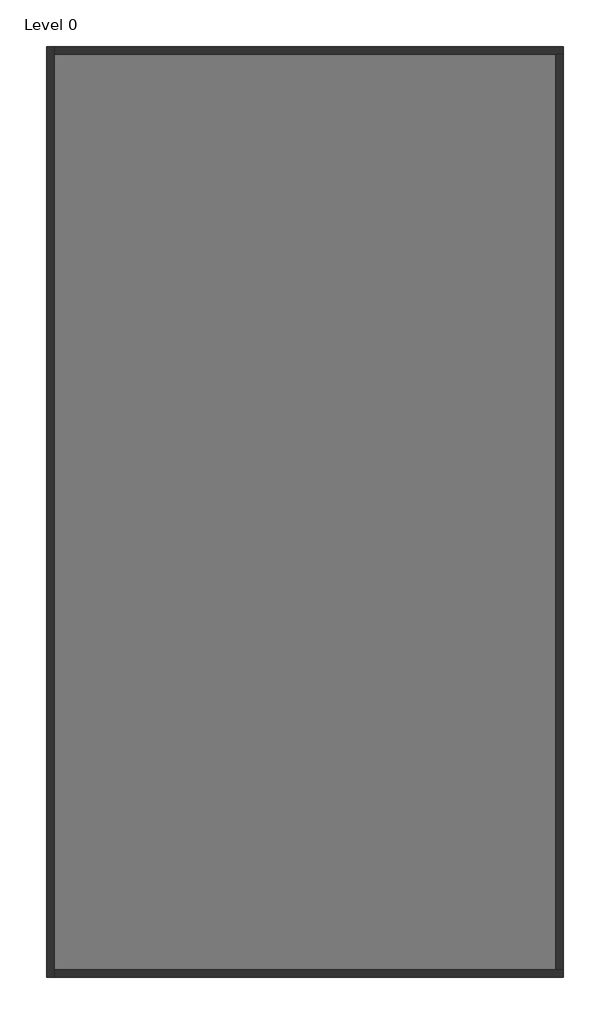
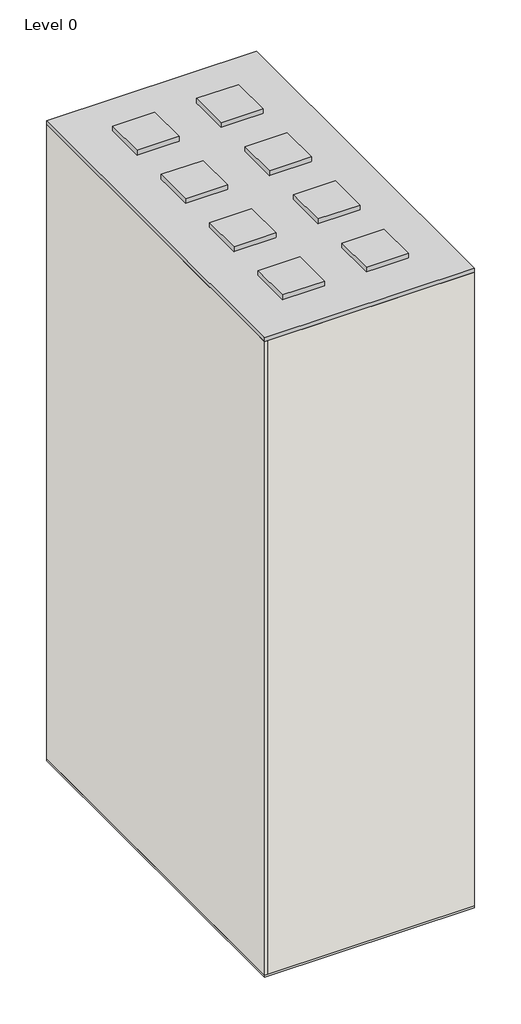
# One storey: 4 walls, 1 proxy, 1 slab.
"""IFC4 building model written with IfcOpenShell, lengths in millimetres."""

from ifc_helpers import new_model, si_unit, frame, origin, origin_with_axes, place, context, project, spatial, polyline, outline, extrude, faceted_brep, element, save

model = new_model("IFC4")

# Units and contexts
model_context = context("Model", 3, world=origin())
ifc_project = project(units=[si_unit("LENGTHUNIT", "METRE", prefix="MILLI")], contexts=[model_context])

# Site, building, storey
site = spatial("IfcSite", under=ifc_project)
building = spatial("IfcBuilding", under=site)
storey = spatial("IfcBuildingStorey", under=building, Name="Level 0", Elevation=100.0)

# Proxy
placement = place(None, origin())
element("IfcBuildingElementProxy", 1, Name="LowUrbanDensityBuilding : LowUrbanDensityBuilding", ObjectType="LowUrbanDensityBuilding : LowUrbanDensityBuilding", at=placement, inside=storey, context=model_context, shape_type="SweptSolid", body=[
    extrude(outline(polyline([(7325.2659446, 3676.2074539), (7325.2659446, -14323.7925461), (-2674.7340554, -14323.7925461), (-2674.7340554, 3676.2074539), (7325.2659446, 3676.2074539)])), origin_with_axes(), (0.0, 0.0, 1.0), 32200.0),
    extrude(outline(polyline([(1325.2659446, 1676.2074539), (1325.2659446, -323.7925461), (-674.7340554, -323.7925461), (-674.7340554, 1676.2074539), (1325.2659446, 1676.2074539)])), frame((0.0, 0.0, 32000.0), z_axis=(0.0, 0.0, 1.0), x_axis=(1.0, 0.0, 0.0)), (0.0, 0.0, 1.0), 445.0),
    extrude(outline(polyline([(3325.2659446, -323.7925461), (3325.2659446, 1676.2074539), (5325.2659446, 1676.2074539), (5325.2659446, -323.7925461), (3325.2659446, -323.7925461)])), frame((0.0, 0.0, 32000.0), z_axis=(0.0, 0.0, 1.0), x_axis=(1.0, 0.0, 0.0)), (0.0, 0.0, 1.0), 445.0),
    extrude(outline(polyline([(1325.2659446, -2323.7925461), (1325.2659446, -4323.7925461), (-674.7340554, -4323.7925461), (-674.7340554, -2323.7925461), (1325.2659446, -2323.7925461)])), frame((0.0, 0.0, 32000.0), z_axis=(0.0, 0.0, 1.0), x_axis=(1.0, 0.0, 0.0)), (0.0, 0.0, 1.0), 445.0),
    extrude(outline(polyline([(3325.2659446, -4323.7925461), (3325.2659446, -2323.7925461), (5325.2659446, -2323.7925461), (5325.2659446, -4323.7925461), (3325.2659446, -4323.7925461)])), frame((0.0, 0.0, 32000.0), z_axis=(0.0, 0.0, 1.0), x_axis=(1.0, 0.0, 0.0)), (0.0, 0.0, 1.0), 445.0),
    extrude(outline(polyline([(-674.7340554, -8323.7925461), (-674.7340554, -6323.7925461), (1325.2659446, -6323.7925461), (1325.2659446, -8323.7925461), (-674.7340554, -8323.7925461)])), frame((0.0, 0.0, 32000.0), z_axis=(0.0, 0.0, 1.0), x_axis=(1.0, 0.0, 0.0)), (0.0, 0.0, 1.0), 445.0),
    extrude(outline(polyline([(3325.2659446, -8323.7925461), (3325.2659446, -6323.7925461), (5325.2659446, -6323.7925461), (5325.2659446, -8323.7925461), (3325.2659446, -8323.7925461)])), frame((0.0, 0.0, 32000.0), z_axis=(0.0, 0.0, 1.0), x_axis=(1.0, 0.0, 0.0)), (0.0, 0.0, 1.0), 445.0),
    extrude(outline(polyline([(-674.7340554, -12323.7925461), (-674.7340554, -10323.7925461), (1325.2659446, -10323.7925461), (1325.2659446, -12323.7925461), (-674.7340554, -12323.7925461)])), frame((0.0, 0.0, 32000.0), z_axis=(0.0, 0.0, 1.0), x_axis=(1.0, 0.0, 0.0)), (0.0, 0.0, 1.0), 445.0),
    extrude(outline(polyline([(5325.2659446, -10323.7925461), (5325.2659446, -12323.7925461), (3325.2659446, -12323.7925461), (3325.2659446, -10323.7925461), (5325.2659446, -10323.7925461)])), frame((0.0, 0.0, 32000.0), z_axis=(0.0, 0.0, 1.0), x_axis=(1.0, 0.0, 0.0)), (0.0, 0.0, 1.0), 445.0),
])

# Slab
element("IfcSlab", 2, ObjectType="Floor-Concrete_100Con", at=placement, inside=storey, context=model_context, shape_type="SweptSolid", body=[
    extrude(outline(polyline([(7325.2659446, 3676.2074539), (7325.2659446, -14323.7925461), (-2674.7340554, -14323.7925461), (-2674.7340554, 3676.2074539), (7325.2659446, 3676.2074539)])), origin_with_axes(), (0.0, 0.0, 1.0), 100.0),
])

# Walls
element("IfcWall", 3, ObjectType="Wall-Ext_25Rdr-100Blk-19P", at=placement, inside=storey, context=model_context, shape_type="Brep", body=[
    faceted_brep([(-2674.7340554, 3676.2074539, 100.0), (-2674.7340554, -14323.7925461, 100.0), (-2674.7340554, -14323.7925461, 32000.0), (-2674.7340554, 3676.2074539, 32000.0), (-2530.4340554, 3676.2074539, 100.0), (-2530.4340554, 3676.2074539, 32000.0), (-2530.4340554, 3531.9074539, 32000.0), (-2530.4340554, -14179.4925461, 32000.0), (-2530.4340554, -14323.7925461, 32000.0), (-2530.4340554, -14323.7925461, 100.0), (-2530.4340554, -14179.4925461, 100.0), (-2530.4340554, 3531.9074539, 100.0)], [[[0, 1, 2, 3]], [[4, 5, 6, 7, 8, 9, 10, 11]], [[1, 0, 4, 11, 10, 9]], [[3, 2, 8, 7, 6, 5]], [[2, 1, 9, 8]], [[0, 3, 5, 4]]]),
])
element("IfcWall", 4, ObjectType="Wall-Ext_25Rdr-100Blk-19P", at=placement, inside=storey, context=model_context, shape_type="Brep", body=[
    faceted_brep([(-2530.4340554, -14323.7925461, 100.0), (7325.2659446, -14323.7925461, 100.0), (7325.2659446, -14323.7925461, 32000.0), (-2530.4340554, -14323.7925461, 32000.0), (-2530.4340554, -14179.4925461, 100.0), (-2530.4340554, -14179.4925461, 32000.0), (7180.9659446, -14179.4925461, 32000.0), (7325.2659446, -14179.4925461, 32000.0), (7325.2659446, -14179.4925461, 100.0), (7180.9659446, -14179.4925461, 100.0)], [[[0, 1, 2, 3]], [[4, 5, 6, 7, 8, 9]], [[1, 0, 4, 9, 8]], [[3, 2, 7, 6, 5]], [[0, 3, 5, 4]], [[2, 1, 8, 7]]]),
])
element("IfcWall", 5, ObjectType="Wall-Ext_25Rdr-100Blk-19P", at=placement, inside=storey, context=model_context, shape_type="Brep", body=[
    faceted_brep([(7325.2659446, 3676.2074539, 100.0), (-2530.4340554, 3676.2074539, 100.0), (-2530.4340554, 3676.2074539, 32000.0), (7325.2659446, 3676.2074539, 32000.0), (7325.2659446, 3531.9074539, 100.0), (7325.2659446, 3531.9074539, 32000.0), (7180.9659446, 3531.9074539, 32000.0), (-2530.4340554, 3531.9074539, 32000.0), (-2530.4340554, 3531.9074539, 100.0), (7180.9659446, 3531.9074539, 100.0)], [[[0, 1, 2, 3]], [[4, 5, 6, 7, 8, 9]], [[1, 0, 4, 9, 8]], [[3, 2, 7, 6, 5]], [[2, 1, 8, 7]], [[0, 3, 5, 4]]]),
])
element("IfcWall", 6, ObjectType="Wall-Ext_25Rdr-100Blk-19P", at=placement, inside=storey, context=model_context, shape_type="SweptSolid", body=[
    extrude(outline(polyline([(7325.2659446, 3531.9074539), (7325.2659446, -14179.4925461), (7180.9659446, -14179.4925461), (7180.9659446, 3531.9074539), (7325.2659446, 3531.9074539)])), frame((0.0, 0.0, 100.0), z_axis=(0.0, 0.0, 1.0), x_axis=(1.0, 0.0, 0.0)), (0.0, 0.0, 1.0), 31900.0),
])

save(model, "model.ifc")

# Revit data of these elements
# Project information
#   Project Issue Date = "Issue Date"
#   Project Status = "Project Status"
#   Client Name = "Owner"
#   Project Address = "Enter address here"
#   Project Name = "Project Name"
#   Project Number = "Project Number"
# Type "Floor-Concrete_100Con"
#   Keynote = "E60/130"
#   Function = 0
#   Layers, outside or top first: 100 mm "Concrete" (function 1)
# Type "Wall-Ext_25Rdr-100Blk-19P"
#   Keynote = "F10"
#   Layers, outside or top first: 25.3 mm "Render, Beige, Smooth" (function 5); 100 mm "Concrete Masonry Units _Low Density" (function 1); 19 mm "Plaster" (function 5)
# Element 1 (IfcBuildingElementProxy, "LowUrbanDensityBuilding : LowUrbanDensityBuilding")
#   Phase Created = New Construction
#   Materials on its faces: "Default Form"
# Element 2 (IfcSlab, "Floor-Concrete_100Con")
#   Height Offset From Level = 0 mm
#   Phase Created = New Construction
#   Materials on its faces: "Concrete"
# Element 3 (IfcWall, "Wall-Ext_25Rdr-100Blk-19P")
#   Top Offset = 0 mm
#   Base Offset = 0 mm
#   wall height = 31900 mm
#   Phase Created = New Construction
#   Base Constraint = Level 0
#   Top Constraint = Level 8
#   Materials on its faces: "Render, Beige, Smooth", "Default Wall", "Plaster"
# Elements 4, 5, 6 (IfcWall, "Wall-Ext_25Rdr-100Blk-19P")
#   Top Offset = 0 mm
#   Base Offset = 0 mm
#   wall height = 31900 mm
#   Phase Created = New Construction
#   Base Constraint = Level 0
#   Top Constraint = Level 8
#   Materials on its faces: "Default Wall", "Render, Beige, Smooth", "Plaster"
# Materials
#   "Concrete": class "Concrete", colour RGB 120 120 120, transparency 0, Description = "Portland Cement Concrete", Cost = 0
#   "Render, Beige, Smooth": class "Generic", colour RGB 213 198 180, transparency 0, Description = "physical material", Cost = 0
#   "Concrete Masonry Units _Low Density": class "Masonry", colour RGB 181 181 181, transparency 0, Description = "Concrete masonry units", Cost = 0
#   "Plaster": class "Generic", colour RGB 249 249 249, transparency 0, Description = "Plaster", Cost = 0
#   "Default Form": class "Generic", colour RGB 185 189 196, transparency 0.5, Cost = 0
#   "Default Wall": class "Miscellaneous", colour RGB 128 128 128, transparency 0, Comments = "Rendering appearance not upgraded Rendering appearance not upgraded ", Cost = 0
